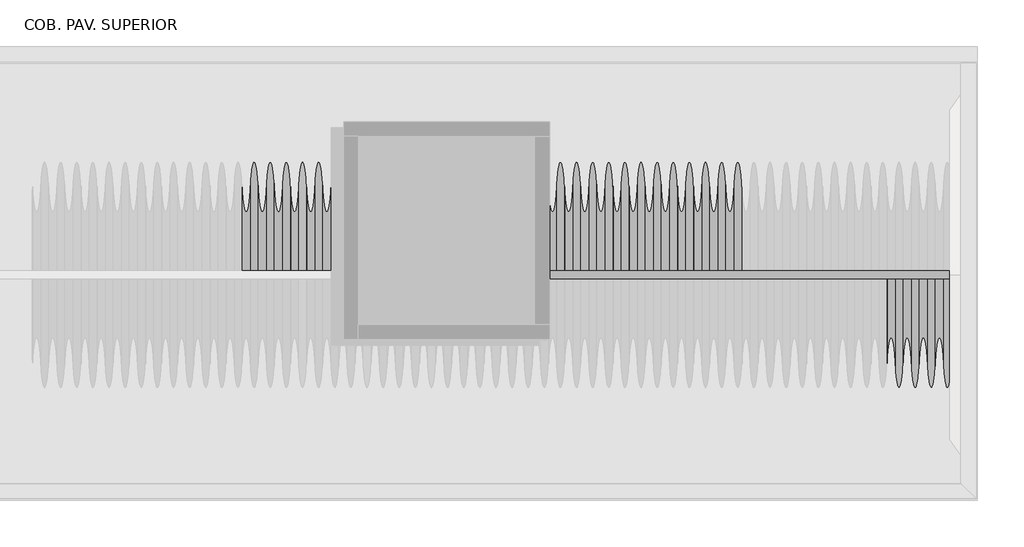
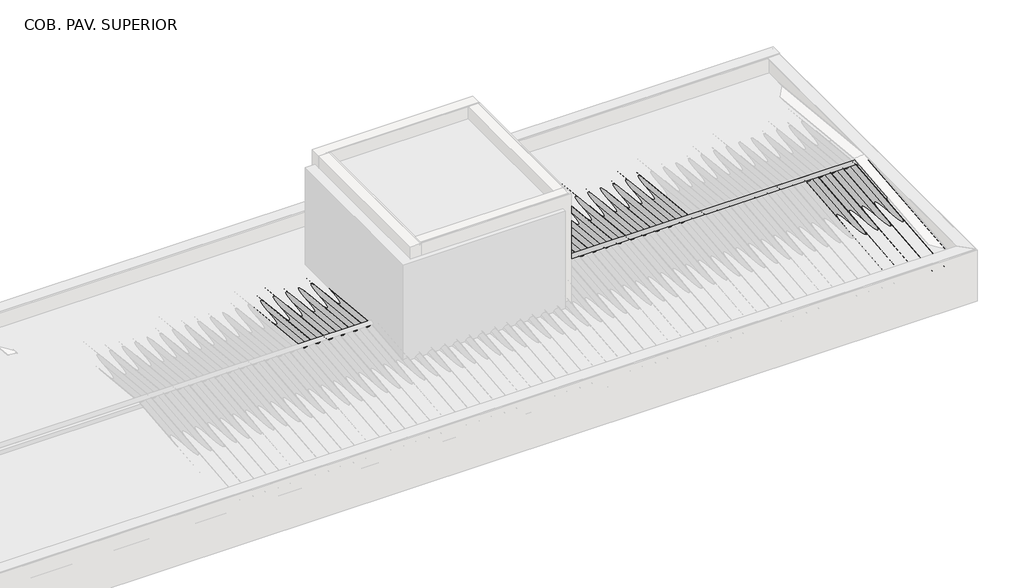
# One storey, part 7 of 8: 46 beams, 8 columns.
# Revit data of these elements (continued)
# Elements 8, 9 (IfcBeam, "Madeira de lei : Berço 6x12cm") (continued)
#   Materials on its faces: ".MADEIRAMENTO"
# Element 10 (IfcBeam, "Madeira de lei : Berço 6x12cm")
#   Comments = ""
#   Uso = "TELHADOS ESTRUTURAS"
#   Compr Cmcl = 3.00 m
#   Structural Material = .MADEIRAMENTO
#   Phase Created = CC_AP
#   Materials on its faces: ".MADEIRAMENTO"
# Element 11 (IfcBeam, "Cumeeira Telha Ondulada : Fibrocimento")
#   Comments = ""
#   Uso = "TELHADOS TELHAS"
#   Phase Created = CC_AP
#   Materials on its faces: ".TELHA DE FIBROCIMENTO"
# Elements 12, 13, 14, 15, 16, 17, 18, 19, 20, 21, 22, 23, 24, 25, 26, 27, 28, 29, 30, 31, 32, 33, 34, 35, 36, 37, 38, 39, 40, 41, 42, 43, 44, 45 (IfcBeam, "Telha Ondulada : Fibrocimento")
#   Uso = "TELHADOS TELHAS"
#   Phase Created = CC_AP
#   Materials on its faces: ".TELHA DE FIBROCIMENTO"
# Element 46 (IfcBeam, "Madeira de lei : Viga Cumeeira 6x16cm")
#   Comments = ""
#   Uso = "TELHADOS MADEIRAMENTO"
#   Compr Cmcl = 6.50 m
#   Structural Material = .MADEIRAMENTO
#   Phase Created = CC_AP
#   Materials on its faces: ".MADEIRAMENTO"
# Elements 47, 48, 49, 50 (IfcColumn, "Madeira de lei-Coluna : Pontalete 6X16cm")
#   Comments = ""
#   Uso = "TELHADOS ESTRUTURAS"
#   Compr Cmcl = 6.00 m
#   Structural Material = .MADEIRAMENTO
#   Phase Created = CC_AP
#   Materials on its faces: ".MADEIRAMENTO"
# Elements 51, 52 (IfcColumn, "Madeira de lei-Coluna : Pontalete 6X16cm")
#   Comments = ""
#   Uso = "TELHADOS ESTRUTURAS"
#   Compr Cmcl = 4.00 m
#   Structural Material = .MADEIRAMENTO
#   Phase Created = CC_AP
#   Materials on its faces: ".MADEIRAMENTO"
# Elements 53, 54 (IfcColumn, "Madeira de lei-Coluna : Pontalete 6X16cm")
#   Comments = ""
#   Uso = "TELHADOS ESTRUTURAS"
#   Compr Cmcl = 5.00 m
#   Structural Material = .MADEIRAMENTO
#   Phase Created = CC_AP
#   Materials on its faces: ".MADEIRAMENTO"
# Materials
#   ".TELHA DE FIBROCIMENTO": class "CC_TELHADO", colour RGB 77 77 76, transparency 0, Description = "TELHA ONDULADA FIBROCIMENTO", Cost = 0
#   ".MADEIRAMENTO": class ".CC_MADEIRAS", colour RGB 212 179 113, transparency 0, Cost = 0
